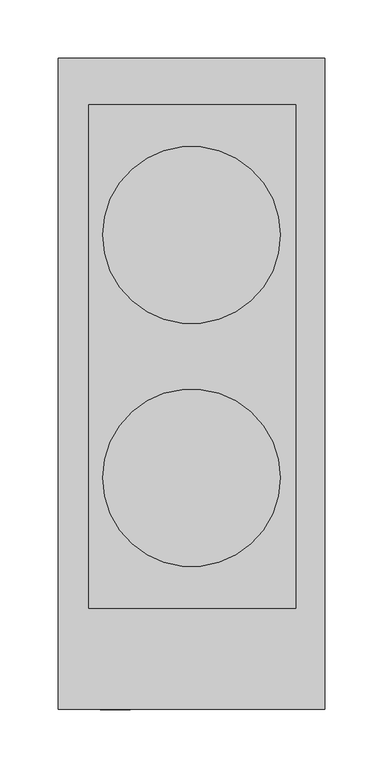
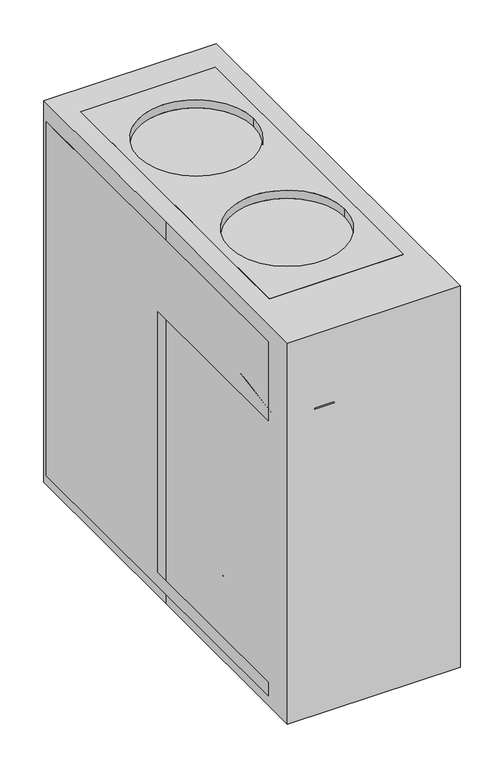
"""IFC4 building model written with IfcOpenShell, lengths in millimetres: proxy geometry, K1552 - Brewer, Coffee, Auto, Elect, 3 Burner, Front-Back : K1552 - Brewer, Coffee, Auto, Elect, 3 Burner, Front-Back."""

import ifcopenshell
import ifcopenshell.guid

model = None  # the IFC model being written
_history = None  # IfcOwnerHistory: only IFC2X3 demands one
_inside = {}  # id of a spatial element -> (the spatial element, [elements in it])
_under = {}  # id of a project, library or spatial element -> (it, [spatial elements below it])
_declared = {}  # id of a project -> (the project, [libraries it declares])
_typed = {}  # id of a type object -> (the type object, [elements of that type])
_made_of = {}  # id of a material, layer set ... -> (it, [elements and type objects made of it])


def new_model(schema):
    """Start an empty IFC model of exactly this schema.

    Asked for "IFC4X3", IfcOpenShell would pick the latest addendum, in which some entities
    have other attributes; the version numbers below select the first issue.
    IFC2X3 requires an IfcOwnerHistory on every rooted entity: one is made here for all.
    """
    global model, _history
    if schema == "IFC4X3":
        model = ifcopenshell.file(schema_version=(4, 3, 0, 0))
    else:
        model = ifcopenshell.file(schema=schema)
    _inside.clear()
    _under.clear()
    _declared.clear()
    _typed.clear()
    _made_of.clear()
    _history = None
    if model.schema == "IFC2X3":
        org = make("IfcOrganization", Name="unknown")
        user = make(
            "IfcPersonAndOrganization",
            ThePerson=make("IfcPerson", FamilyName="unknown"),
            TheOrganization=org,
        )
        app = make(
            "IfcApplication",
            ApplicationDeveloper=org,
            Version="unknown",
            ApplicationFullName="unknown",
            ApplicationIdentifier="unknown",
        )
        _history = make(
            "IfcOwnerHistory",
            OwningUser=user,
            OwningApplication=app,
            ChangeAction="ADDED",
            CreationDate=0,
        )
    return model


def make(cls, **values):
    """One entity of the class cls with the attributes given. An attribute that is None is left unset."""
    return model.create_entity(
        cls, **{name: value for name, value in values.items() if value is not None}
    )


def rooted(cls, **values):
    """An entity with a GlobalId (a new one), such as an element, a storey or a relation."""
    return make(cls, GlobalId=ifcopenshell.guid.new(), OwnerHistory=_history, **values)


def si_unit(unit_type, name, prefix=None):
    """IfcSIUnit, for example si_unit("LENGTHUNIT", "METRE", prefix="MILLI")."""
    return make("IfcSIUnit", UnitType=unit_type, Prefix=prefix, Name=name)


def assignment(units):
    """IfcUnitAssignment: the units of a project."""
    return None if units is None else make("IfcUnitAssignment", Units=units)


def point(xyz):
    """IfcCartesianPoint."""
    return None if xyz is None else make("IfcCartesianPoint", Coordinates=xyz)


def direction(xyz):
    """IfcDirection."""
    return None if xyz is None else make("IfcDirection", DirectionRatios=xyz)


def frame(location, z_axis=None, x_axis=None):
    """IfcAxis2Placement3D, a coordinate frame: its origin and axes. An axis left out is left unset."""
    return make(
        "IfcAxis2Placement3D",
        Location=point(location),
        Axis=direction(z_axis),
        RefDirection=direction(x_axis),
    )


def frame_2d(location, x_axis=None):
    """IfcAxis2Placement2D, a coordinate frame in the plane: its origin and x axis."""
    return make(
        "IfcAxis2Placement2D", Location=point(location), RefDirection=direction(x_axis)
    )


def origin():
    """The frame at (0, 0, 0) with its axes left unset."""
    return frame((0.0, 0.0, 0.0))


def origin_with_axes():
    """The frame at (0, 0, 0) with the z axis (0, 0, 1) and the x axis (1, 0, 0) written out."""
    return frame((0.0, 0.0, 0.0), z_axis=(0.0, 0.0, 1.0), x_axis=(1.0, 0.0, 0.0))


def place(relative_to, where):
    """IfcLocalPlacement: puts the frame where relative to a parent placement (None: the world)."""
    return make(
        "IfcLocalPlacement", PlacementRelTo=relative_to, RelativePlacement=where
    )


def context(
    kind, dimensions, precision=None, world=None, true_north=None, identifier=None
):
    """IfcGeometricRepresentationContext, for example the 3D "Model" context."""
    return make(
        "IfcGeometricRepresentationContext",
        ContextIdentifier=identifier,
        ContextType=kind,
        CoordinateSpaceDimension=dimensions,
        Precision=precision,
        WorldCoordinateSystem=world,
        TrueNorth=true_north,
    )


def project(units=None, contexts=None):
    """IfcProject with its units and contexts."""
    return rooted(
        "IfcProject",
        Name="project",
        RepresentationContexts=contexts,
        UnitsInContext=assignment(units),
    )


def spatial(cls, under=None, at=None, **own):
    """A site, building, storey or space (cls), placed at a placement, below another one or the project."""
    s = rooted(cls, ObjectPlacement=at, **own)
    if under is not None:
        _under.setdefault(under.id(), (under, []))[1].append(s)
    return s


def polyline(points):
    """IfcPolyline through the points."""
    return make("IfcPolyline", Points=[point(p) for p in points])


def circle_curve(where, radius):
    """IfcCircle in the frame where."""
    return make("IfcCircle", Position=where, Radius=radius)


def ellipse_curve(where, semi_axis1, semi_axis2):
    """IfcEllipse in the frame where."""
    return make(
        "IfcEllipse", Position=where, SemiAxis1=semi_axis1, SemiAxis2=semi_axis2
    )


def trimmed(basis, trim1, trim2, sense, master):
    """IfcTrimmedCurve: the piece of a basis curve between two trims."""
    return make(
        "IfcTrimmedCurve",
        BasisCurve=basis,
        Trim1=trim1,
        Trim2=trim2,
        SenseAgreement=sense,
        MasterRepresentation=master,
    )


def segment(curve, same_sense, transition):
    """IfcCompositeCurveSegment."""
    return make(
        "IfcCompositeCurveSegment",
        Transition=transition,
        SameSense=same_sense,
        ParentCurve=curve,
    )


def composite_curve(segments, self_intersect=None):
    """IfcCompositeCurve: segments joined end to end."""
    return make("IfcCompositeCurve", Segments=segments, SelfIntersect=self_intersect)


def outline(outer, holes=None, kind="AREA"):
    """IfcArbitraryClosedProfileDef: a profile drawn as a closed curve; with holes, ...WithVoids."""
    if holes is None:
        return make("IfcArbitraryClosedProfileDef", ProfileType=kind, OuterCurve=outer)
    return make(
        "IfcArbitraryProfileDefWithVoids",
        ProfileType=kind,
        OuterCurve=outer,
        InnerCurves=holes,
    )


def extrude(swept, where, along, depth):
    """IfcExtrudedAreaSolid: the profile swept, set in the frame where, extruded along a direction by depth."""
    return make(
        "IfcExtrudedAreaSolid",
        SweptArea=swept,
        Position=where,
        ExtrudedDirection=direction(along),
        Depth=depth,
    )


def shape(context_of_items, identifier, shape_type, items):
    """IfcShapeRepresentation: the items that make up one representation, for example the "Body"."""
    return make(
        "IfcShapeRepresentation",
        ContextOfItems=context_of_items,
        RepresentationIdentifier=identifier,
        RepresentationType=shape_type,
        Items=items,
    )


def source(mapping_origin, context_of_items, identifier, shape_type, items):
    """IfcRepresentationMap: a shape defined once, which mapped items show again and again."""
    return make(
        "IfcRepresentationMap",
        MappingOrigin=mapping_origin,
        MappedRepresentation=shape(context_of_items, identifier, shape_type, items),
    )


def transform(
    local_origin,
    x_axis=None,
    y_axis=None,
    z_axis=None,
    scale=None,
    scale2=None,
    scale3=None,
    uniform=True,
):
    """IfcCartesianTransformationOperator3D, or its non-uniform kind. x_axis, y_axis, z_axis: its Axis1, 2, 3."""
    if uniform:
        return make(
            "IfcCartesianTransformationOperator3D",
            Axis1=direction(x_axis),
            Axis2=direction(y_axis),
            LocalOrigin=point(local_origin),
            Scale=scale,
            Axis3=direction(z_axis),
        )
    return make(
        "IfcCartesianTransformationOperator3DnonUniform",
        Axis1=direction(x_axis),
        Axis2=direction(y_axis),
        LocalOrigin=point(local_origin),
        Scale=scale,
        Axis3=direction(z_axis),
        Scale2=scale2,
        Scale3=scale3,
    )


def mapped(mapping_source, mapping_target):
    """IfcMappedItem: shows the shape of a source again, moved by a transform."""
    return make(
        "IfcMappedItem", MappingSource=mapping_source, MappingTarget=mapping_target
    )


def made_of(thing, what):
    """Note that an element or type object is made of a material, layer set ...; save() writes the relation."""
    if what is not None:
        _made_of.setdefault(what.id(), (what, []))[1].append(thing)
    return thing


def element(
    cls,
    number,
    at=None,
    inside=None,
    cuts=None,
    type_object=None,
    material=None,
    context=None,
    identifier="Body",
    shape_type=None,
    held_by="IfcProductDefinitionShape",
    body=None,
    shapes=None,
    **own,
):
    """One element of the class cls, such as IfcWall. Its Tag is "e" and its number.

    at: its placement. inside: the storey or other place that contains it. cuts: it is an
    opening in that element (IfcRelVoidsElement). A single representation is given by context,
    identifier, shape_type and body (its items); several are given by shapes. held_by: the class
    of the entity that holds the representations. save() writes the other relations.
    """
    e = rooted(cls, Tag="e%d" % number, ObjectPlacement=at, **own)
    if body is not None:
        shapes = [shape(context, identifier, shape_type, body)]
    if shapes is not None:
        e.Representation = make(held_by, Representations=shapes)
    if inside is not None:
        _inside.setdefault(inside.id(), (inside, []))[1].append(e)
    if cuts is not None:
        rooted(
            "IfcRelVoidsElement", RelatingBuildingElement=cuts, RelatedOpeningElement=e
        )
    if type_object is not None:
        _typed.setdefault(type_object.id(), (type_object, []))[1].append(e)
    return made_of(e, material)


def aggregate(whole, parts):
    """IfcRelAggregates: a whole, such as a stair, and the parts it consists of."""
    return rooted("IfcRelAggregates", RelatingObject=whole, RelatedObjects=parts)


def save(model, path):
    """Write the relations noted so far, then the file.

    IfcRelAggregates (storeys below a building ...), IfcRelContainedInSpatialStructure (elements
    in a storey), IfcRelDefinesByType, IfcRelAssociatesMaterial and IfcRelDeclares: one each for
    every whole, place, type object, material and project.
    """
    for whole, parts in _under.values():
        aggregate(whole, parts)
    for where, things in _inside.values():
        rooted(
            "IfcRelContainedInSpatialStructure",
            RelatedElements=things,
            RelatingStructure=where,
        )
    for kind, things in _typed.values():
        rooted("IfcRelDefinesByType", RelatedObjects=things, RelatingType=kind)
    for what, things in _made_of.values():
        rooted("IfcRelAssociatesMaterial", RelatedObjects=things, RelatingMaterial=what)
    for by, libraries in _declared.values():
        rooted("IfcRelDeclares", RelatingContext=by, RelatedDefinitions=libraries)
    model.write(path)


def plane_surface(at):
    """IfcPlane: the flat surface through the origin of the frame at, square to its z axis."""
    return make("IfcPlane", Position=at)


def cylinder_surface(at, radius):
    """IfcCylindricalSurface: all points at the distance radius from the z axis of the frame at."""
    return make("IfcCylindricalSurface", Position=at, Radius=radius)


def revolved_surface(curve, axis_point, axis_direction):
    """IfcSurfaceOfRevolution: the curve turned about the line through axis_point along axis_direction."""
    return make(
        "IfcSurfaceOfRevolution",
        SweptCurve=make("IfcArbitraryOpenProfileDef", ProfileType="CURVE", Curve=curve),
        AxisPosition=make("IfcAxis1Placement", Location=point(axis_point), Axis=direction(axis_direction)),
    )


def advanced_brep(points, edges, surfaces, faces):
    """IfcAdvancedBrep: a solid bounded by faces that lie on surfaces and meet in shared edges.

    An edge is (start, end): straight between two places in points (the first is 0);
    or (start, end, curve); or (start, end, curve, False) where it runs against its curve.
    A face is (place in surfaces, loops), or (place, loops, False) where it looks against
    its surface's normal. A loop lists edges by number (the first is 1), with a minus sign
    where the edge is run from its end to its start. The first loop is the outer one.
    """
    corners = [point(p) for p in points]
    vertices = [make("IfcVertexPoint", VertexGeometry=c) for c in corners]
    made = []
    for start, end, *more in edges:
        made.append(
            make(
                "IfcEdgeCurve",
                EdgeStart=vertices[start],
                EdgeEnd=vertices[end],
                EdgeGeometry=more[0] if more else make("IfcPolyline", Points=[corners[start], corners[end]]),
                SameSense=more[1] if len(more) > 1 else True,
            )
        )
    hull = []
    for where, loops, *sense in faces:
        bounds = []
        for j, loop in enumerate(loops):
            ring = [make("IfcOrientedEdge", EdgeElement=made[abs(k) - 1], Orientation=k > 0) for k in loop]
            bounds.append(
                make(
                    "IfcFaceOuterBound" if j == 0 else "IfcFaceBound",
                    Bound=make("IfcEdgeLoop", EdgeList=ring),
                    Orientation=True,
                )
            )
        hull.append(make("IfcAdvancedFace", Bounds=bounds, FaceSurface=surfaces[where], SameSense=sense[0] if sense else True))
    return make("IfcAdvancedBrep", Outer=make("IfcClosedShell", CfsFaces=hull))


def specialty_equipment_200fc004(model_context):
    return source(origin(), model_context, "Body", "SolidModel", [
        extrude(outline(polyline([(-6.35, 0.0), (6.35, 0.0), (13.7065038, -50.8), (-11.6934962, -50.8), (-6.35, 0.0)])), frame((-66.3573194, -248.7924454, 469.1875481), z_axis=(0.0, -0.866025403784439, 0.49999999999999944), x_axis=(1.0, 0.0, 0.0)), (0.0, 0.0, 1.0), 6.35),
        extrude(outline(polyline([(-60.0073194, -247.65), (-72.7073194, -247.65), (-72.7073194, -234.95), (-60.0073194, -234.95), (-60.0073194, -247.65)])), frame((0.0, 0.0, 456.4875481), z_axis=(0.0, 0.0, 1.0), x_axis=(1.0, 0.0, 0.0)), (0.0, 0.0, 1.0), 12.7),
        extrude(outline(polyline([(99.1586716, -247.65), (54.7086716, -247.65), (54.7086716, -234.95), (99.1586716, -234.95), (99.1586716, -247.65)])), frame((0.0, 0.0, 482.1172372), z_axis=(0.0, 0.0, 1.0), x_axis=(1.0, 0.0, 0.0)), (0.0, 0.0, 1.0), 12.7),
        extrude(outline(polyline([(35.6586716, -247.65), (-8.7913284, -247.65), (-8.7913284, -234.95), (35.6586716, -234.95), (35.6586716, -247.65)])), frame((0.0, 0.0, 482.1172372), z_axis=(0.0, 0.0, 1.0), x_axis=(1.0, 0.0, 0.0)), (0.0, 0.0, 1.0), 12.7),
        extrude(outline(composite_curve([segment(trimmed(circle_curve(frame_2d((449.9890787, 64.52786)), 6.35), [point((449.9890787, 58.17786))], [point((449.9890787, 70.87786))], False, "CARTESIAN"), True, "CONTINUOUS"), segment(trimmed(circle_curve(frame_2d((449.9890787, 64.52786)), 6.35), [point((449.9890787, 70.87786))], [point((449.9890787, 58.17786))], False, "CARTESIAN"), True, "CONTINUOUS")], self_intersect=False)), frame((0.0, -247.65, 0.0), z_axis=(0.0, 1.0, 0.0), x_axis=(0.0, 0.0, 1.0)), (0.0, 0.0, 1.0), 12.7),
        extrude(outline(composite_curve([segment(trimmed(circle_curve(frame_2d((449.9890787, 26.42786)), 6.35), [point((449.9890787, 20.07786))], [point((449.9890787, 32.77786))], False, "CARTESIAN"), True, "CONTINUOUS"), segment(trimmed(circle_curve(frame_2d((449.9890787, 26.42786)), 6.35), [point((449.9890787, 32.77786))], [point((449.9890787, 20.07786))], False, "CARTESIAN"), True, "CONTINUOUS")], self_intersect=False)), frame((0.0, -247.65, 0.0), z_axis=(0.0, 1.0, 0.0), x_axis=(0.0, 0.0, 1.0)), (0.0, 0.0, 1.0), 12.7),
        advanced_brep(
        [(-76.2, 127.7134023, 522.1626312), (76.2, 127.7134023, 522.1626312), (-76.2, 127.7134023, 533.4), (76.2, 127.7134023, 533.4), (-76.2, -80.7485258, 522.1626312), (76.2, -80.7485258, 522.1626312), (-76.2, -80.7485258, 533.4), (76.2, -80.7485258, 533.4), (89.4998195, 239.3021594, 533.4), (-88.3001805, 239.3021594, 533.4), (-88.3001805, -192.4978406, 533.4), (89.4998195, -192.4978406, 533.4), (89.4998195, 239.3021594, 508.0), (89.4998195, -192.4978406, 508.0), (-88.3001805, -192.4978406, 508.0), (-88.3001805, 239.3021594, 508.0)],
        [
            (0, 1, circle_curve(frame((0.0, 127.7134023, 522.1626312), z_axis=(0.0, 0.0, 1.0), x_axis=(1.0, 0.0, 0.0)), 76.2)),
            (1, 0, circle_curve(frame((0.0, 127.7134023, 522.1626312), z_axis=(0.0, 0.0, 1.0), x_axis=(1.0, 0.0, 0.0)), 76.2)),
            (0, 2),
            (2, 3, circle_curve(frame((0.0, 127.7134023, 533.4), z_axis=(0.0, 0.0, 1.0), x_axis=(1.0, 0.0, 0.0)), 76.2)),
            (3, 1),
            (3, 2, circle_curve(frame((0.0, 127.7134023, 533.4), z_axis=(0.0, 0.0, 1.0), x_axis=(1.0, 0.0, 0.0)), 76.2)),
            (4, 5, circle_curve(frame((0.0, -80.7485258, 522.1626312), z_axis=(0.0, 0.0, 1.0), x_axis=(1.0, 0.0, 0.0)), 76.2)),
            (5, 4, circle_curve(frame((0.0, -80.7485258, 522.1626312), z_axis=(0.0, 0.0, 1.0), x_axis=(1.0, 0.0, 0.0)), 76.2)),
            (4, 6),
            (6, 7, circle_curve(frame((0.0, -80.7485258, 533.4), z_axis=(0.0, 0.0, 1.0), x_axis=(1.0, 0.0, 0.0)), 76.2)),
            (7, 5),
            (7, 6, circle_curve(frame((0.0, -80.7485258, 533.4), z_axis=(0.0, 0.0, 1.0), x_axis=(1.0, 0.0, 0.0)), 76.2)),
            (8, 9),
            (9, 10),
            (10, 11),
            (11, 8),
            (12, 13),
            (13, 14),
            (14, 15),
            (15, 12),
            (8, 12),
            (15, 9),
            (14, 10),
            (13, 11),
        ],
        [
            plane_surface(frame((76.2, 127.7134023, 522.1626312), z_axis=(0.0, 0.0, 1.0), x_axis=(0.0, -1.0, 0.0))),
            revolved_surface(polyline([(76.2, 127.7134023, 533.4), (76.2, 127.7134023, 522.1626312)]), (0.0, 127.7134023, 522.1626312), (0.0, 0.0, 1.0)),
            plane_surface(frame((76.2, -80.7485258, 522.1626312), z_axis=(0.0, 0.0, 1.0), x_axis=(0.0, -1.0, 0.0))),
            revolved_surface(polyline([(76.2, -80.7485258, 533.4), (76.2, -80.7485258, 522.1626312)]), (0.0, -80.7485258, 522.1626312), (0.0, 0.0, 1.0)),
            plane_surface(frame((-69.2501805, 239.3021594, 533.4), z_axis=(0.0, 0.0, 1.0), x_axis=(-1.0, 0.0, 0.0))),
            plane_surface(frame((-69.2501805, 239.3021594, 508.0), z_axis=(0.0, 0.0, -1.0), x_axis=(1.0, 0.0, 0.0))),
            plane_surface(frame((89.4998195, 239.3021594, 533.4), z_axis=(0.0, 1.0, 0.0), x_axis=(0.0, 0.0, -1.0))),
            plane_surface(frame((-88.3001805, 239.3021594, 533.4), z_axis=(-1.0, 0.0, 0.0), x_axis=(0.0, 0.0, -1.0))),
            plane_surface(frame((-88.3001805, -192.4978406, 533.4), z_axis=(0.0, -1.0, 0.0), x_axis=(0.0, 0.0, -1.0))),
            plane_surface(frame((89.4998195, -192.4978406, 533.4), z_axis=(1.0, 0.0, 0.0), x_axis=(0.0, 0.0, -1.0))),
        ],
        [
            (0, [[1, 2]]),
            (1, [[-1, 3, 4, 5]]),
            (1, [[-2, -5, 6, -3]]),
            (2, [[7, 8]]),
            (3, [[-7, 9, 10, 11]]),
            (3, [[-8, -11, 12, -9]]),
            (4, [[13, 14, 15, 16], [-4, -6], [-10, -12]]),
            (5, [[17, 18, 19, 20]]),
            (6, [[-13, 21, -20, 22]]),
            (7, [[-14, -22, -19, 23]]),
            (8, [[-15, -23, -18, 24]]),
            (9, [[-16, -24, -17, -21]]),
        ],
    ),
        extrude(outline(polyline([(-234.95, 12.7), (-234.95, 31.75), (19.05, 31.75), (19.05, 397.4233361), (-234.95, 397.4233361), (-234.95, 508.0), (273.05, 508.0), (273.05, 12.7), (-234.95, 12.7)])), frame((-114.3, 0.0, 0.0), z_axis=(1.0, 0.0, 0.0), x_axis=(0.0, 1.0, 0.0)), (0.0, 0.0, 1.0), 228.6),
        advanced_brep(
        [(-114.3, 279.4, 533.4), (-114.3, 0.0, 533.4), (-114.3, -279.4, 533.4), (114.3, -279.4, 533.4), (114.3, 279.4, 533.4), (76.2, 127.7134023, 533.4), (-76.2, 127.7134023, 533.4), (76.2, -80.7485258, 533.4), (-76.2, -80.7485258, 533.4), (-114.3, 279.4, 0.0), (114.3, 279.4, 0.0), (114.3, -279.4, 0.0), (-114.3, -279.4, 0.0), (-114.3, 0.0, 0.0), (-76.2, 127.7134023, 522.1626312), (76.2, 127.7134023, 522.1626312), (-76.2, -80.7485258, 522.1626312), (76.2, -80.7485258, 522.1626312)],
        [
            (0, 1),
            (1, 2),
            (2, 3),
            (3, 4),
            (4, 0),
            (5, 6, circle_curve(frame((0.0, 127.7134023, 533.4), z_axis=(0.0, 0.0, -1.0), x_axis=(1.0, 0.0, 0.0)), 76.2)),
            (6, 5, circle_curve(frame((0.0, 127.7134023, 533.4), z_axis=(0.0, 0.0, -1.0), x_axis=(1.0, 0.0, 0.0)), 76.2)),
            (7, 8, circle_curve(frame((0.0, -80.7485258, 533.4), z_axis=(0.0, 0.0, -1.0), x_axis=(1.0, 0.0, 0.0)), 76.2)),
            (8, 7, circle_curve(frame((0.0, -80.7485258, 533.4), z_axis=(0.0, 0.0, -1.0), x_axis=(1.0, 0.0, 0.0)), 76.2)),
            (9, 10),
            (10, 11),
            (11, 12),
            (12, 13),
            (13, 9),
            (0, 9),
            (13, 1),
            (12, 2),
            (11, 3),
            (10, 4),
            (14, 15, circle_curve(frame((0.0, 127.7134023, 522.1626312), z_axis=(0.0, 0.0, 1.0), x_axis=(1.0, 0.0, 0.0)), 76.2)),
            (15, 14, circle_curve(frame((0.0, 127.7134023, 522.1626312), z_axis=(0.0, 0.0, 1.0), x_axis=(1.0, 0.0, 0.0)), 76.2)),
            (14, 6),
            (5, 15),
            (16, 17, circle_curve(frame((0.0, -80.7485258, 522.1626312), z_axis=(0.0, 0.0, 1.0), x_axis=(1.0, 0.0, 0.0)), 76.2)),
            (17, 16, circle_curve(frame((0.0, -80.7485258, 522.1626312), z_axis=(0.0, 0.0, 1.0), x_axis=(1.0, 0.0, 0.0)), 76.2)),
            (16, 8),
            (7, 17),
        ],
        [
            plane_surface(frame((-114.3, 0.0, 533.4), z_axis=(0.0, 0.0, 1.0), x_axis=(0.0, -1.0, 0.0))),
            plane_surface(frame((-114.3, 0.0, 0.0), z_axis=(0.0, 0.0, -1.0), x_axis=(0.0, 1.0, 0.0))),
            plane_surface(frame((-114.3, 279.4, 533.4), z_axis=(-1.0, 0.0, 0.0), x_axis=(0.0, 0.0, -1.0))),
            plane_surface(frame((-114.3, 0.0, 533.4), z_axis=(-1.0, 0.0, 0.0), x_axis=(0.0, 0.0, -1.0))),
            plane_surface(frame((-114.3, -279.4, 533.4), z_axis=(0.0, -1.0, 0.0), x_axis=(0.0, 0.0, -1.0))),
            plane_surface(frame((114.3, -279.4, 533.4), z_axis=(1.0, 0.0, 0.0), x_axis=(0.0, 0.0, -1.0))),
            plane_surface(frame((114.3, 279.4, 533.4), z_axis=(0.0, 1.0, 0.0), x_axis=(0.0, 0.0, -1.0))),
            plane_surface(frame((76.2, 127.7134023, 522.1626312), z_axis=(0.0, 0.0, 1.0), x_axis=(0.0, -1.0, 0.0))),
            revolved_surface(polyline([(76.2, 127.7134023, 533.4), (76.2, 127.7134023, 522.1626312)]), (0.0, 127.7134023, 522.1626312), (0.0, 0.0, 1.0)),
            plane_surface(frame((76.2, -80.7485258, 522.1626312), z_axis=(0.0, 0.0, 1.0), x_axis=(0.0, -1.0, 0.0))),
            revolved_surface(polyline([(76.2, -80.7485258, 533.4), (76.2, -80.7485258, 522.1626312)]), (0.0, -80.7485258, 522.1626312), (0.0, 0.0, 1.0)),
        ],
        [
            (0, [[1, 2, 3, 4, 5], [6, 7], [8, 9]]),
            (1, [[10, 11, 12, 13, 14]]),
            (2, [[-1, 15, -14, 16]]),
            (3, [[-2, -16, -13, 17]]),
            (4, [[-3, -17, -12, 18]]),
            (5, [[-4, -18, -11, 19]]),
            (6, [[-5, -19, -10, -15]]),
            (7, [[20, 21]]),
            (8, [[-20, 22, -6, 23]]),
            (8, [[-21, -23, -7, -22]]),
            (9, [[24, 25]]),
            (10, [[-24, 26, -8, 27]]),
            (10, [[-25, -27, -9, -26]]),
        ],
    ),
        advanced_brep(
        [(-12.9117986, -140.1635833, 258.171536), (13.4227125, -140.1635833, 258.171536), (13.4227125, -146.5135833, 247.1730134), (-12.9117986, -146.5135833, 247.1730134), (13.4227125, -178.6584125, 280.396536), (13.4227125, -222.4331171, 272.6778745), (13.4227125, -266.5280753, 163.5390233), (13.4227125, -254.7528403, 158.7815196), (13.4227125, -211.4999829, 265.8360982), (13.4227125, -185.0084125, 269.3980134), (-12.9117986, -185.0084125, 269.3980134), (-12.9117986, -211.4999829, 265.8360982), (-12.9117986, -254.7528403, 158.7815196), (-12.9117986, -266.5280753, 163.5390233), (-12.9117986, -222.4331171, 272.6778745), (-12.9117986, -178.6584125, 280.396536), (0.0, -178.6584125, 280.396536), (0.0, -222.4331171, 272.6778745)],
        [
            (0, 1),
            (1, 2),
            (2, 3),
            (3, 0),
            (1, 4),
            (4, 5, circle_curve(frame((13.4227125, -195.9463935, 250.4528745), z_axis=(1.0, 0.0, 0.0), x_axis=(0.0, 0.5000000000000018, 0.8660254037844376)), 34.5759621)),
            (5, 6),
            (6, 7),
            (7, 8),
            (8, 9, circle_curve(frame((13.4227125, -195.9463935, 250.4528745), z_axis=(-1.0, 0.0, 0.0), x_axis=(0.0, 0.5000000000000018, 0.8660254037844376)), 21.8759621)),
            (9, 2),
            (9, 10),
            (10, 3),
            (10, 11, circle_curve(frame((-12.9117986, -195.9463935, 250.4528745), z_axis=(1.0, 0.0, 0.0), x_axis=(0.0, 0.5000000000000018, 0.8660254037844376)), 21.8759621)),
            (11, 12),
            (12, 13),
            (13, 14),
            (14, 15, circle_curve(frame((-12.9117986, -195.9463935, 250.4528745), z_axis=(-1.0, 0.0, 0.0), x_axis=(0.0, 0.5000000000000018, 0.8660254037844376)), 34.5759621)),
            (15, 0),
            (15, 16),
            (16, 4),
            (8, 11),
            (17, 16, circle_curve(frame((0.0, -195.9463935, 250.4528745), z_axis=(-1.0, 0.0, 0.0), x_axis=(0.0, 0.5000000000000018, 0.8660254037844376)), 34.5759621)),
            (14, 17),
            (17, 5),
            (6, 13),
            (12, 7),
        ],
        [
            plane_surface(frame((0.0, -140.1635833, 258.171536), z_axis=(0.0, 0.8660254037844374, -0.5000000000000023), x_axis=(1.0, 0.0, 0.0))),
            plane_surface(frame((13.4227125, -140.1635833, 258.171536), z_axis=(1.0, 0.0, 0.0), x_axis=(0.0, -0.8660254037844374, 0.5000000000000023))),
            plane_surface(frame((13.4227125, -146.5135833, 247.1730134), z_axis=(0.0, -0.5000000000000026, -0.8660254037844373), x_axis=(0.0, -0.8660254037844373, 0.5000000000000026))),
            plane_surface(frame((-12.9117986, -146.5135833, 247.1730134), z_axis=(-1.0, 0.0, 0.0), x_axis=(0.0, -0.8660254037844373, 0.5000000000000026))),
            plane_surface(frame((0.0, -140.1635833, 258.171536), z_axis=(0.0, 0.5000000000000023, 0.8660254037844374), x_axis=(0.0, -0.8660254037844374, 0.5000000000000023))),
            revolved_surface(polyline([(13.4227125, -185.00841244999995, 269.39801341082557), (-12.9117986, -185.00841244999995, 269.39801341082557)]), (0.0, -195.9463935, 250.4528745), (1.0, 0.0, 0.0)),
            cylinder_surface(frame((0.0, -195.9463935, 250.4528745), z_axis=(1.0, 0.0, 0.0), x_axis=(0.0, 0.5000000000000018, 0.8660254037844376)), 34.5759621),
            plane_surface(frame((0.0, -266.5280753, 163.5390233), z_axis=(0.0, -0.3746065934159136, -0.9271838545667869), x_axis=(1.0, 0.0, 0.0))),
            plane_surface(frame((13.4227125, -211.4999829, 265.8360982), z_axis=(0.0, 0.9271838545667866, -0.3746065934159138), x_axis=(0.0, -0.3746065934159138, -0.9271838545667866))),
            plane_surface(frame((0.0, -222.4331171, 272.6778745), z_axis=(0.0, -0.9271838545667866, 0.37460659341591407), x_axis=(0.0, -0.37460659341591407, -0.9271838545667866))),
        ],
        [
            (0, [[1, 2, 3, 4]]),
            (1, [[-2, 5, 6, 7, 8, 9, 10, 11]]),
            (2, [[-3, -11, 12, 13]]),
            (3, [[-4, -13, 14, 15, 16, 17, 18, 19]]),
            (4, [[-19, 20, 21, -5, -1]]),
            (5, [[-14, -12, -10, 22]]),
            (6, [[23, -20, -18, 24]]),
            (6, [[-6, -21, -23, 25]]),
            (7, [[26, -16, 27, -8]]),
            (8, [[-22, -9, -27, -15]]),
            (9, [[-25, -24, -17, -26, -7]]),
        ],
    ),
        advanced_brep(
        [(0.0, -181.2530218, 222.25), (0.0, -54.2530218, 222.25), (0.0, -54.2530218, 44.45), (0.0, -181.2530218, 44.45), (0.0, -146.1023815, 249.80937), (0.0, -89.4036621, 249.80937), (0.0, -146.1023815, 262.50937), (0.0, -89.4036621, 262.50937), (0.0, -179.0936518, 295.5006403), (0.0, -56.4123918, 295.5006403), (0.0, -117.7530218, 295.5006403), (0.0, -117.7530218, 44.45)],
        [
            (0, 1, circle_curve(frame((0.0, -117.7530218, 222.25), z_axis=(0.0, 0.0, -1.0), x_axis=(0.0, 1.0, 0.0)), 63.5)),
            (1, 2, circle_curve(frame((0.0, -123.9538288, 133.35), z_axis=(-1.0, 0.0, 0.0), x_axis=(0.0, 1.0, 0.0)), 112.966422)),
            (2, 3, circle_curve(frame((0.0, -117.7530218, 44.45), z_axis=(0.0, 0.0, 1.0), x_axis=(0.0, 1.0, 0.0)), 63.5)),
            (3, 0, circle_curve(frame((0.0, -111.5522148, 133.35), z_axis=(-1.0, 0.0, 0.0), x_axis=(0.0, -1.0, 0.0)), 112.966422)),
            (1, 0, circle_curve(frame((0.0, -117.7530218, 222.25), z_axis=(0.0, 0.0, -1.0), x_axis=(0.0, 1.0, 0.0)), 63.5)),
            (3, 2, circle_curve(frame((0.0, -117.7530218, 44.45), z_axis=(0.0, 0.0, 1.0), x_axis=(0.0, 1.0, 0.0)), 63.5)),
            (4, 5, circle_curve(frame((0.0, -117.7530218, 249.80937), z_axis=(0.0, 0.0, -1.0), x_axis=(0.0, 1.0, 0.0)), 28.3493597)),
            (5, 1),
            (0, 4),
            (5, 4, circle_curve(frame((0.0, -117.7530218, 249.80937), z_axis=(0.0, 0.0, -1.0), x_axis=(0.0, 1.0, 0.0)), 28.3493597)),
            (6, 7, circle_curve(frame((0.0, -117.7530218, 262.50937), z_axis=(0.0, 0.0, -1.0), x_axis=(0.0, 1.0, 0.0)), 28.3493597)),
            (7, 5),
            (4, 6),
            (7, 6, circle_curve(frame((0.0, -117.7530218, 262.50937), z_axis=(0.0, 0.0, -1.0), x_axis=(0.0, 1.0, 0.0)), 28.3493597)),
            (8, 9, circle_curve(frame((0.0, -117.7530218, 295.5006403), z_axis=(0.0, 0.0, -1.0), x_axis=(0.0, 1.0, 0.0)), 61.34063)),
            (9, 7),
            (6, 8),
            (9, 8, circle_curve(frame((0.0, -117.7530218, 295.5006403), z_axis=(0.0, 0.0, -1.0), x_axis=(0.0, 1.0, 0.0)), 61.34063)),
            (10, 9),
            (8, 10),
            (2, 11),
            (11, 3),
        ],
        [
            revolved_surface(trimmed(ellipse_curve(frame((0.0, -123.9538288, 133.35), z_axis=(1.0, 0.0, 0.0), x_axis=(0.0, 1.0, 0.0)), 112.966422, 112.966422), [point((0.0, -54.2530218, 44.45))], [point((0.0, -54.2530218, 222.25))], True, "CARTESIAN"), (0.0, -117.7530218, 444.5), (0.0, 0.0, 1.0)),
            revolved_surface(polyline([(0.0, -54.2530218, 222.25), (0.0, -89.4036621, 249.80937)]), (0.0, -117.7530218, 444.5), (0.0, 0.0, 1.0)),
            cylinder_surface(frame((0.0, -117.7530218, 444.5), z_axis=(0.0, 0.0, 1.0), x_axis=(0.0, 1.0, 0.0)), 28.3493597),
            revolved_surface(polyline([(0.0, -89.4036621, 262.50937), (0.0, -56.4123918, 295.5006403)]), (0.0, -117.7530218, 444.5), (0.0, 0.0, 1.0)),
            plane_surface(frame((0.0, -117.7530218, 295.5006403), z_axis=(0.0, 0.0, 1.0), x_axis=(0.0, 1.0, 0.0))),
            plane_surface(frame((0.0, -117.7530218, 44.45), z_axis=(0.0, 0.0, -1.0), x_axis=(0.0, 1.0, 0.0))),
        ],
        [
            (0, [[1, 2, 3, 4]]),
            (0, [[5, -4, 6, -2]]),
            (1, [[7, 8, -1, 9]]),
            (1, [[10, -9, -5, -8]]),
            (2, [[11, 12, -7, 13]]),
            (2, [[14, -13, -10, -12]]),
            (3, [[15, 16, -11, 17]]),
            (3, [[18, -17, -14, -16]]),
            (4, [[19, -15, 20]]),
            (4, [[-20, -18, -19]]),
            (5, [[-3, 21, 22]]),
            (5, [[-6, -22, -21]]),
        ],
    ),
        advanced_brep(
        [(-76.2, -117.7530218, 370.4823042), (76.2, -117.7530218, 370.4823042), (-38.1, -117.7530218, 305.756644), (38.1, -117.7530218, 305.756644)],
        [
            (0, 1, circle_curve(frame((0.0, -117.7530218, 370.4823042), z_axis=(0.0, 0.0, 1.0), x_axis=(-1.0, 0.0, 0.0)), 76.2)),
            (1, 0, circle_curve(frame((0.0, -117.7530218, 370.4823042), z_axis=(0.0, 0.0, 1.0), x_axis=(1.0, 0.0, 0.0)), 76.2)),
            (2, 3, circle_curve(frame((0.0, -117.7530218, 305.756644), z_axis=(0.0, 0.0, -1.0), x_axis=(1.0, 0.0, 0.0)), 38.1)),
            (3, 2, circle_curve(frame((0.0, -117.7530218, 305.756644), z_axis=(0.0, 0.0, -1.0), x_axis=(-1.0, 0.0, 0.0)), 38.1)),
            (3, 1),
            (0, 2),
        ],
        [
            plane_surface(frame((0.0, -117.7530218, 370.4823042), z_axis=(0.0, 0.0, 1.0), x_axis=(0.0, -1.0, 0.0))),
            plane_surface(frame((0.0, -117.7530218, 305.756644), z_axis=(0.0, 0.0, -1.0), x_axis=(0.0, -1.0, 0.0))),
            revolved_surface(polyline([(38.09999997056809, -117.7530218, 305.756644), (76.2, -117.7530218, 370.4823042)]), (0.0, -117.7530218, 241.0309839), (0.0, 0.0, 1.0)),
            revolved_surface(polyline([(-38.09999997056809, -117.7530218, 305.756644), (-76.2, -117.7530218, 370.4823042)]), (0.0, -117.7530218, 241.0309839), (0.0, 0.0, 1.0)),
        ],
        [
            (0, [[1, 2]]),
            (1, [[3, 4]]),
            (2, [[-4, 5, -1, 6]]),
            (3, [[-3, -6, -2, -5]]),
        ],
    ),
        extrude(outline(composite_curve([segment(trimmed(circle_curve(frame_2d((0.0, -117.7530218)), 76.2), [point((-76.2, -117.7530218))], [point((76.2, -117.7530218))], False, "CARTESIAN"), True, "CONTINUOUS"), segment(trimmed(circle_curve(frame_2d((0.0, -117.7530218)), 76.2), [point((76.2, -117.7530218))], [point((-76.2, -117.7530218))], False, "CARTESIAN"), True, "CONTINUOUS")], self_intersect=False)), frame((0.0, 0.0, 370.4823042), z_axis=(0.0, 0.0, 1.0), x_axis=(1.0, 0.0, 0.0)), (0.0, 0.0, 1.0), 26.9410319),
        extrude(outline(composite_curve([segment(trimmed(circle_curve(frame_2d((82.683617, 53.3907009)), 6.35), [point((89.033617, 53.3907009))], [point((76.333617, 53.3907009))], False, "CARTESIAN"), True, "CONTINUOUS"), segment(trimmed(circle_curve(frame_2d((82.683617, 53.3907009)), 6.35), [point((76.333617, 53.3907009))], [point((89.033617, 53.3907009))], False, "CARTESIAN"), True, "CONTINUOUS")], self_intersect=False)), origin_with_axes(), (0.0, 0.0, 1.0), 12.7),
        extrude(outline(composite_curve([segment(trimmed(circle_curve(frame_2d((-82.683617, 53.3907009)), 6.35), [point((-89.033617, 53.3907009))], [point((-76.333617, 53.3907009))], False, "CARTESIAN"), True, "CONTINUOUS"), segment(trimmed(circle_curve(frame_2d((-82.683617, 53.3907009)), 6.35), [point((-76.333617, 53.3907009))], [point((-89.033617, 53.3907009))], False, "CARTESIAN"), True, "CONTINUOUS")], self_intersect=False)), origin_with_axes(), (0.0, 0.0, 1.0), 12.7),
        extrude(outline(composite_curve([segment(trimmed(circle_curve(frame_2d((0.0, -117.7530218)), 76.2), [point((-76.2, -117.7530218))], [point((76.2, -117.7530218))], False, "CARTESIAN"), True, "CONTINUOUS"), segment(trimmed(circle_curve(frame_2d((0.0, -117.7530218)), 76.2), [point((76.2, -117.7530218))], [point((-76.2, -117.7530218))], False, "CARTESIAN"), True, "CONTINUOUS")], self_intersect=False)), frame((0.0, 0.0, 31.75), z_axis=(0.0, 0.0, 1.0), x_axis=(1.0, 0.0, 0.0)), (0.0, 0.0, 1.0), 12.7),
        extrude(outline(composite_curve([segment(trimmed(circle_curve(frame_2d((82.683617, -200.6092991)), 6.35), [point((89.033617, -200.6092991))], [point((76.333617, -200.6092991))], False, "CARTESIAN"), True, "CONTINUOUS"), segment(trimmed(circle_curve(frame_2d((82.683617, -200.6092991)), 6.35), [point((76.333617, -200.6092991))], [point((89.033617, -200.6092991))], False, "CARTESIAN"), True, "CONTINUOUS")], self_intersect=False)), origin_with_axes(), (0.0, 0.0, 1.0), 12.7),
        extrude(outline(composite_curve([segment(trimmed(circle_curve(frame_2d((-82.683617, -200.6092991)), 6.35), [point((-89.033617, -200.6092991))], [point((-76.333617, -200.6092991))], False, "CARTESIAN"), True, "CONTINUOUS"), segment(trimmed(circle_curve(frame_2d((-82.683617, -200.6092991)), 6.35), [point((-76.333617, -200.6092991))], [point((-89.033617, -200.6092991))], False, "CARTESIAN"), True, "CONTINUOUS")], self_intersect=False)), origin_with_axes(), (0.0, 0.0, 1.0), 12.7),
        extrude(outline(composite_curve([segment(trimmed(circle_curve(frame_2d((82.683617, 243.8907009)), 6.35), [point((89.033617, 243.8907009))], [point((76.333617, 243.8907009))], False, "CARTESIAN"), True, "CONTINUOUS"), segment(trimmed(circle_curve(frame_2d((82.683617, 243.8907009)), 6.35), [point((76.333617, 243.8907009))], [point((89.033617, 243.8907009))], False, "CARTESIAN"), True, "CONTINUOUS")], self_intersect=False)), origin_with_axes(), (0.0, 0.0, 1.0), 12.7),
        extrude(outline(composite_curve([segment(trimmed(circle_curve(frame_2d((-82.683617, 243.8907009)), 6.35), [point((-89.033617, 243.8907009))], [point((-76.333617, 243.8907009))], False, "CARTESIAN"), True, "CONTINUOUS"), segment(trimmed(circle_curve(frame_2d((-82.683617, 243.8907009)), 6.35), [point((-76.333617, 243.8907009))], [point((-89.033617, 243.8907009))], False, "CARTESIAN"), True, "CONTINUOUS")], self_intersect=False)), origin_with_axes(), (0.0, 0.0, 1.0), 12.7),
    ])


if __name__ == "__main__":
    model = new_model("IFC4")
    model_context = context("Model", 3, world=origin())
    ifc_project = project(units=[si_unit("LENGTHUNIT", "METRE", prefix="MILLI")], contexts=[model_context])
    site = spatial("IfcSite", under=ifc_project)
    building = spatial("IfcBuilding", under=site)
    placement = place(None, origin())
    specialty_equipment_shape = specialty_equipment_200fc004(model_context)
    element("IfcBuildingElementProxy", 1, Name="K1552 - Brewer, Coffee, Auto, Elect, 3 Burner, Front-Back : K1552 - Brewer, Coffee, Auto, Elect, 3 Burner, Front-Back", ObjectType="K1552 - Brewer, Coffee, Auto, Elect, 3 Burner, Front-Back : K1552 - Brewer, Coffee, Auto, Elect, 3 Burner, Front-Back", at=placement, inside=building, context=model_context, shape_type="MappedRepresentation", body=[
        mapped(specialty_equipment_shape, transform((0.0, 0.0, 0.0), x_axis=(1.0, 0.0, 0.0), y_axis=(0.0, 1.0, 0.0), z_axis=(0.0, 0.0, 1.0))),
    ])
    save(model, "model.ifc")

# Revit data of these elements
# Project information
#   Sheets - Total = "5"
#   Project Issue Date = "Issue Date"
#   Project Status = "Project Status"
#   Client Name = "Owner"
#   Project Address = "Enter address here"
#   Project Name = "Project Name"
#   Project Number = "Project Number"
#   Publication Date = "30-Jan-15"
# Type "K1552 - Brewer, Coffee, Auto, Elect, 3 Burner, Front-Back : K1552 - Brewer, Coffee, Auto, Elect, 3 Burner, Front-Back"
#   Watts2 = "0"
#   Watts1 = "1800"
#   Unit_Issue = "EA"
#   UTIL_6_Misc = "-"
#   UTIL_5_NonMedGas = "-"
#   UTIL_4_MiscGas = "-"
#   UTIL_3_MedGas = "-"
#   UTIL_2_Elec = "A"
#   UTIL_1_WaterDrain = "J"
#   Nomenclature = "Brewer, Coffee, Auto, Elect, 3 Burner, Front/Back"
#   NSN = "7310"
#   Location [instance default] = ""
#   JSN = "K1552"
#   Fund_Source_VA = "-"
#   Fund_Source_Navy = "-"
#   Fund_Source_Army = "-"
#   Fund_Source_AF = "-"
#   ELEC_Volts2 = "0"
#   ELEC_Volts1 = "120"
#   ELEC_Phase2 = "0"
#   ELEC_Phase1 = "1"
#   ELEC_HertzSwitch = "0"
#   ELEC_HertzDependent = "-1"
#   ELEC_Hertz = "60"
#   ELEC_Amps2 = "0"
#   ELEC_Amps1 = "15"
#   DetailDescription = "Space saving front to back automatic coffee maker. This unit includes a heating tank, connection for a cold water supply, decanter service with three burners, funnel and a water flow controller. The unit is used for semi-automatic coffee brewing in cafeterias and commercial institutions. The unit automatically shuts off the water flow when enough has passed through to fill the pot. The unit is normally provided plumbed with a hot water faucet to the side for making other hot drinks (tea, cider, cocoa, etc.). The database height dimension does not include the clearance for coffee decanters warming on the upper burners."
#   CAT_VA = "C"
#   CAT_Navy = "C"
#   CAT_IHS = "-"
#   CAT_Army = "C"
#   CAT_AF = "C"
#   BTUperhour = "0"
#   Weight_IP = 37
#   DIM_Width_IP = 0' - 9"
#   DIM_Height_IP = 1' - 9"
#   DIM_Depth_IP = 1' - 10"
# Element 1 (IfcBuildingElementProxy, "K1552 - Brewer, Coffee, Auto, Elect, 3 Burner, Front-Back : K1552 - Brewer, Coffee, Auto, Elect, 3 Burner, Front-Back")
#   Location = "NCWD1"
#   Materials on its faces: "EquipSpace"
# Materials
#   "EquipSpace": class "Unassigned", colour RGB 221 217 195, transparency 0.5
